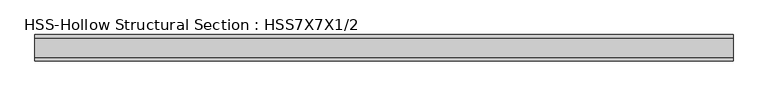
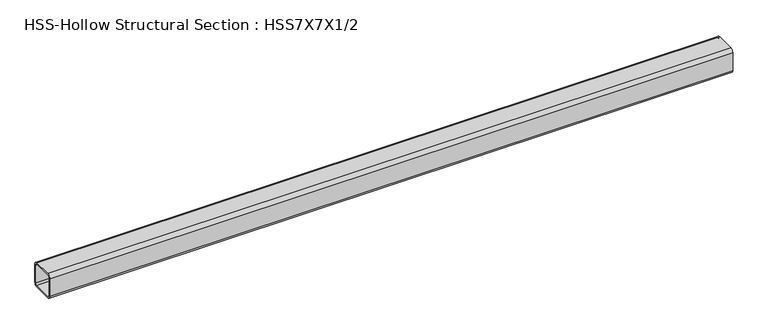
"""IFC4 building model written with IfcOpenShell, lengths in millimetres: member geometry, HSS-Hollow Structural Section : HSS7X7X1/2."""

from ifc_helpers import new_model, si_unit, point, frame, frame_2d, origin, place, context, project, spatial, polyline, circle_curve, trimmed, segment, composite_curve, outline, extrude, source, transform, mapped, element, save


def hss_hollow_structural_section_hss7x7x1_2_daed7586(model_context):
    return source(origin(), model_context, "Body", "SweptSolid", [
        extrude(outline(composite_curve([segment(polyline([(88.9, 65.278), (88.9, -65.278)]), True, "CONTINUOUS"), segment(trimmed(circle_curve(frame_2d((65.278, -65.278)), 23.622), [point((88.9, -65.278))], [point((65.278, -88.9))], False, "CARTESIAN"), True, "CONTINUOUS"), segment(polyline([(65.278, -88.9), (-65.278, -88.9)]), True, "CONTINUOUS"), segment(trimmed(circle_curve(frame_2d((-65.278, -65.278)), 23.622), [point((-65.278, -88.9))], [point((-88.9, -65.278))], False, "CARTESIAN"), True, "CONTINUOUS"), segment(polyline([(-88.9, -65.278), (-88.9, 65.278)]), True, "CONTINUOUS"), segment(trimmed(circle_curve(frame_2d((-65.278, 65.278)), 23.622), [point((-88.9, 65.278))], [point((-65.278, 88.9))], False, "CARTESIAN"), True, "CONTINUOUS"), segment(polyline([(-65.278, 88.9), (65.278, 88.9)]), True, "CONTINUOUS"), segment(trimmed(circle_curve(frame_2d((65.278, 65.278)), 23.622), [point((65.278, 88.9))], [point((88.9, 65.278))], False, "CARTESIAN"), True, "CONTINUOUS")], self_intersect=False), holes=[composite_curve([segment(trimmed(circle_curve(frame_2d((-65.278, 65.278)), 11.811), [point((-65.278, 77.089))], [point((-77.089, 65.278))], True, "CARTESIAN"), True, "CONTINUOUS"), segment(polyline([(-77.089, 65.278), (-77.089, -65.278)]), True, "CONTINUOUS"), segment(trimmed(circle_curve(frame_2d((-65.278, -65.278)), 11.811), [point((-77.089, -65.278))], [point((-65.278, -77.089))], True, "CARTESIAN"), True, "CONTINUOUS"), segment(polyline([(-65.278, -77.089), (65.278, -77.089)]), True, "CONTINUOUS"), segment(trimmed(circle_curve(frame_2d((65.278, -65.278)), 11.811), [point((65.278, -77.089))], [point((77.089, -65.278))], True, "CARTESIAN"), True, "CONTINUOUS"), segment(polyline([(77.089, -65.278), (77.089, 65.278)]), True, "CONTINUOUS"), segment(trimmed(circle_curve(frame_2d((65.278, 65.278)), 11.811), [point((77.089, 65.278))], [point((65.278, 77.089))], True, "CARTESIAN"), True, "CONTINUOUS"), segment(polyline([(65.278, 77.089), (-65.278, 77.089)]), True, "CONTINUOUS")], self_intersect=False)]), frame((-2583.6098476, 0.0, 0.0), z_axis=(1.0, 0.0, 0.0), x_axis=(0.0, 1.0, 0.0)), (0.0, 0.0, 1.0), 4736.9581081),
    ])


if __name__ == "__main__":
    model = new_model("IFC4")
    model_context = context("Model", 3, world=origin())
    ifc_project = project(units=[si_unit("LENGTHUNIT", "METRE", prefix="MILLI")], contexts=[model_context])
    site = spatial("IfcSite", under=ifc_project)
    building = spatial("IfcBuilding", under=site)
    placement = place(None, origin())
    hss_hollow_structural_section_hss7x7x1_2_shape = hss_hollow_structural_section_hss7x7x1_2_daed7586(model_context)
    element("IfcMember", 1, ObjectType="HSS-Hollow Structural Section : HSS7X7X1/2", at=placement, inside=building, context=model_context, shape_type="MappedRepresentation", body=[
        mapped(hss_hollow_structural_section_hss7x7x1_2_shape, transform((0.0, 0.0, 0.0), x_axis=(1.0, 0.0, 0.0), y_axis=(0.0, 1.0, 0.0), z_axis=(0.0, 0.0, 1.0))),
    ])
    save(model, "model.ifc")

# Revit data of these elements
# Type "HSS-Hollow Structural Section : HSS7X7X1/2"
#   Assembly Code = "B10"
#   Shape = "Square"
#   W = 41.9
#   Ht = 0' - 7"
#   Length [instance default] = 5' - 0"
#   b = 0' - 7"
#   kr = 0' - 0.93"
#   t = 0' - 0.465"
#   A = 0.0805556 SF
#   Structural Material [instance default] = Steel ASTM A500, Grade B, Rectangular and Square
# Element 1 (IfcMember, "HSS-Hollow Structural Section : HSS7X7X1/2")
#   Materials on its faces: "Steel ASTM A500, Grade B, Rectangular and Square"
# Materials
#   "Steel ASTM A500, Grade B, Rectangular and Square": class "Metal", colour RGB 199 199 199, transparency 0, Description = "Carbon steel", Cost = 0
